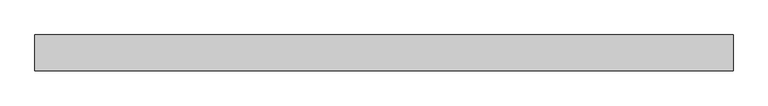
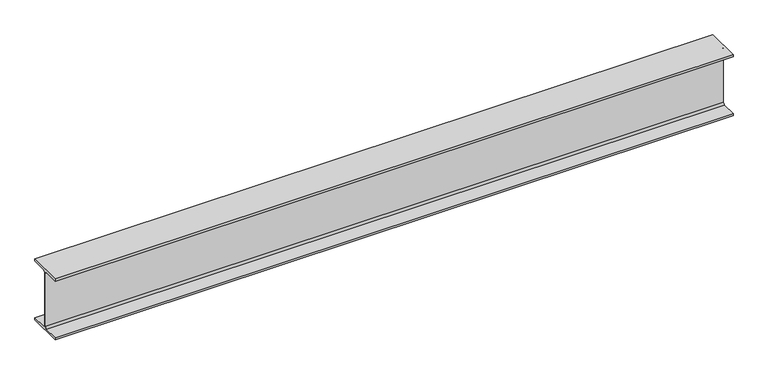
"""IFC4 building model written with IfcOpenShell, lengths in millimetres: beam geometry, Steel Beam_H-KSD3502 : H_SB_ASB_H-200x200x8x12."""

import ifcopenshell
import ifcopenshell.guid

model = None  # the IFC model being written
_history = None  # IfcOwnerHistory: only IFC2X3 demands one
_inside = {}  # id of a spatial element -> (the spatial element, [elements in it])
_under = {}  # id of a project, library or spatial element -> (it, [spatial elements below it])
_declared = {}  # id of a project -> (the project, [libraries it declares])
_typed = {}  # id of a type object -> (the type object, [elements of that type])
_made_of = {}  # id of a material, layer set ... -> (it, [elements and type objects made of it])


def new_model(schema):
    """Start an empty IFC model of exactly this schema.

    Asked for "IFC4X3", IfcOpenShell would pick the latest addendum, in which some entities
    have other attributes; the version numbers below select the first issue.
    IFC2X3 requires an IfcOwnerHistory on every rooted entity: one is made here for all.
    """
    global model, _history
    if schema == "IFC4X3":
        model = ifcopenshell.file(schema_version=(4, 3, 0, 0))
    else:
        model = ifcopenshell.file(schema=schema)
    _inside.clear()
    _under.clear()
    _declared.clear()
    _typed.clear()
    _made_of.clear()
    _history = None
    if model.schema == "IFC2X3":
        org = make("IfcOrganization", Name="unknown")
        user = make(
            "IfcPersonAndOrganization",
            ThePerson=make("IfcPerson", FamilyName="unknown"),
            TheOrganization=org,
        )
        app = make(
            "IfcApplication",
            ApplicationDeveloper=org,
            Version="unknown",
            ApplicationFullName="unknown",
            ApplicationIdentifier="unknown",
        )
        _history = make(
            "IfcOwnerHistory",
            OwningUser=user,
            OwningApplication=app,
            ChangeAction="ADDED",
            CreationDate=0,
        )
    return model


def make(cls, **values):
    """One entity of the class cls with the attributes given. An attribute that is None is left unset."""
    return model.create_entity(
        cls, **{name: value for name, value in values.items() if value is not None}
    )


def rooted(cls, **values):
    """An entity with a GlobalId (a new one), such as an element, a storey or a relation."""
    return make(cls, GlobalId=ifcopenshell.guid.new(), OwnerHistory=_history, **values)


def si_unit(unit_type, name, prefix=None):
    """IfcSIUnit, for example si_unit("LENGTHUNIT", "METRE", prefix="MILLI")."""
    return make("IfcSIUnit", UnitType=unit_type, Prefix=prefix, Name=name)


def assignment(units):
    """IfcUnitAssignment: the units of a project."""
    return None if units is None else make("IfcUnitAssignment", Units=units)


def point(xyz):
    """IfcCartesianPoint."""
    return None if xyz is None else make("IfcCartesianPoint", Coordinates=xyz)


def direction(xyz):
    """IfcDirection."""
    return None if xyz is None else make("IfcDirection", DirectionRatios=xyz)


def frame(location, z_axis=None, x_axis=None):
    """IfcAxis2Placement3D, a coordinate frame: its origin and axes. An axis left out is left unset."""
    return make(
        "IfcAxis2Placement3D",
        Location=point(location),
        Axis=direction(z_axis),
        RefDirection=direction(x_axis),
    )


def frame_2d(location, x_axis=None):
    """IfcAxis2Placement2D, a coordinate frame in the plane: its origin and x axis."""
    return make(
        "IfcAxis2Placement2D", Location=point(location), RefDirection=direction(x_axis)
    )


def origin():
    """The frame at (0, 0, 0) with its axes left unset."""
    return frame((0.0, 0.0, 0.0))


def place(relative_to, where):
    """IfcLocalPlacement: puts the frame where relative to a parent placement (None: the world)."""
    return make(
        "IfcLocalPlacement", PlacementRelTo=relative_to, RelativePlacement=where
    )


def context(
    kind, dimensions, precision=None, world=None, true_north=None, identifier=None
):
    """IfcGeometricRepresentationContext, for example the 3D "Model" context."""
    return make(
        "IfcGeometricRepresentationContext",
        ContextIdentifier=identifier,
        ContextType=kind,
        CoordinateSpaceDimension=dimensions,
        Precision=precision,
        WorldCoordinateSystem=world,
        TrueNorth=true_north,
    )


def project(units=None, contexts=None):
    """IfcProject with its units and contexts."""
    return rooted(
        "IfcProject",
        Name="project",
        RepresentationContexts=contexts,
        UnitsInContext=assignment(units),
    )


def spatial(cls, under=None, at=None, **own):
    """A site, building, storey or space (cls), placed at a placement, below another one or the project."""
    s = rooted(cls, ObjectPlacement=at, **own)
    if under is not None:
        _under.setdefault(under.id(), (under, []))[1].append(s)
    return s


def polyline(points):
    """IfcPolyline through the points."""
    return make("IfcPolyline", Points=[point(p) for p in points])


def circle_curve(where, radius):
    """IfcCircle in the frame where."""
    return make("IfcCircle", Position=where, Radius=radius)


def trimmed(basis, trim1, trim2, sense, master):
    """IfcTrimmedCurve: the piece of a basis curve between two trims."""
    return make(
        "IfcTrimmedCurve",
        BasisCurve=basis,
        Trim1=trim1,
        Trim2=trim2,
        SenseAgreement=sense,
        MasterRepresentation=master,
    )


def segment(curve, same_sense, transition):
    """IfcCompositeCurveSegment."""
    return make(
        "IfcCompositeCurveSegment",
        Transition=transition,
        SameSense=same_sense,
        ParentCurve=curve,
    )


def composite_curve(segments, self_intersect=None):
    """IfcCompositeCurve: segments joined end to end."""
    return make("IfcCompositeCurve", Segments=segments, SelfIntersect=self_intersect)


def outline(outer, holes=None, kind="AREA"):
    """IfcArbitraryClosedProfileDef: a profile drawn as a closed curve; with holes, ...WithVoids."""
    if holes is None:
        return make("IfcArbitraryClosedProfileDef", ProfileType=kind, OuterCurve=outer)
    return make(
        "IfcArbitraryProfileDefWithVoids",
        ProfileType=kind,
        OuterCurve=outer,
        InnerCurves=holes,
    )


def extrude(swept, where, along, depth):
    """IfcExtrudedAreaSolid: the profile swept, set in the frame where, extruded along a direction by depth."""
    return make(
        "IfcExtrudedAreaSolid",
        SweptArea=swept,
        Position=where,
        ExtrudedDirection=direction(along),
        Depth=depth,
    )


def shape(context_of_items, identifier, shape_type, items):
    """IfcShapeRepresentation: the items that make up one representation, for example the "Body"."""
    return make(
        "IfcShapeRepresentation",
        ContextOfItems=context_of_items,
        RepresentationIdentifier=identifier,
        RepresentationType=shape_type,
        Items=items,
    )


def source(mapping_origin, context_of_items, identifier, shape_type, items):
    """IfcRepresentationMap: a shape defined once, which mapped items show again and again."""
    return make(
        "IfcRepresentationMap",
        MappingOrigin=mapping_origin,
        MappedRepresentation=shape(context_of_items, identifier, shape_type, items),
    )


def transform(
    local_origin,
    x_axis=None,
    y_axis=None,
    z_axis=None,
    scale=None,
    scale2=None,
    scale3=None,
    uniform=True,
):
    """IfcCartesianTransformationOperator3D, or its non-uniform kind. x_axis, y_axis, z_axis: its Axis1, 2, 3."""
    if uniform:
        return make(
            "IfcCartesianTransformationOperator3D",
            Axis1=direction(x_axis),
            Axis2=direction(y_axis),
            LocalOrigin=point(local_origin),
            Scale=scale,
            Axis3=direction(z_axis),
        )
    return make(
        "IfcCartesianTransformationOperator3DnonUniform",
        Axis1=direction(x_axis),
        Axis2=direction(y_axis),
        LocalOrigin=point(local_origin),
        Scale=scale,
        Axis3=direction(z_axis),
        Scale2=scale2,
        Scale3=scale3,
    )


def mapped(mapping_source, mapping_target):
    """IfcMappedItem: shows the shape of a source again, moved by a transform."""
    return make(
        "IfcMappedItem", MappingSource=mapping_source, MappingTarget=mapping_target
    )


def made_of(thing, what):
    """Note that an element or type object is made of a material, layer set ...; save() writes the relation."""
    if what is not None:
        _made_of.setdefault(what.id(), (what, []))[1].append(thing)
    return thing


def element(
    cls,
    number,
    at=None,
    inside=None,
    cuts=None,
    type_object=None,
    material=None,
    context=None,
    identifier="Body",
    shape_type=None,
    held_by="IfcProductDefinitionShape",
    body=None,
    shapes=None,
    **own,
):
    """One element of the class cls, such as IfcWall. Its Tag is "e" and its number.

    at: its placement. inside: the storey or other place that contains it. cuts: it is an
    opening in that element (IfcRelVoidsElement). A single representation is given by context,
    identifier, shape_type and body (its items); several are given by shapes. held_by: the class
    of the entity that holds the representations. save() writes the other relations.
    """
    e = rooted(cls, Tag="e%d" % number, ObjectPlacement=at, **own)
    if body is not None:
        shapes = [shape(context, identifier, shape_type, body)]
    if shapes is not None:
        e.Representation = make(held_by, Representations=shapes)
    if inside is not None:
        _inside.setdefault(inside.id(), (inside, []))[1].append(e)
    if cuts is not None:
        rooted(
            "IfcRelVoidsElement", RelatingBuildingElement=cuts, RelatedOpeningElement=e
        )
    if type_object is not None:
        _typed.setdefault(type_object.id(), (type_object, []))[1].append(e)
    return made_of(e, material)


def aggregate(whole, parts):
    """IfcRelAggregates: a whole, such as a stair, and the parts it consists of."""
    return rooted("IfcRelAggregates", RelatingObject=whole, RelatedObjects=parts)


def save(model, path):
    """Write the relations noted so far, then the file.

    IfcRelAggregates (storeys below a building ...), IfcRelContainedInSpatialStructure (elements
    in a storey), IfcRelDefinesByType, IfcRelAssociatesMaterial and IfcRelDeclares: one each for
    every whole, place, type object, material and project.
    """
    for whole, parts in _under.values():
        aggregate(whole, parts)
    for where, things in _inside.values():
        rooted(
            "IfcRelContainedInSpatialStructure",
            RelatedElements=things,
            RelatingStructure=where,
        )
    for kind, things in _typed.values():
        rooted("IfcRelDefinesByType", RelatedObjects=things, RelatingType=kind)
    for what, things in _made_of.values():
        rooted("IfcRelAssociatesMaterial", RelatedObjects=things, RelatingMaterial=what)
    for by, libraries in _declared.values():
        rooted("IfcRelDeclares", RelatingContext=by, RelatedDefinitions=libraries)
    model.write(path)


def beam_0bb79bd1(model_context):
    return source(origin(), model_context, "Body", "SweptSolid", [
        extrude(outline(composite_curve([segment(polyline([(82.5, -141.5), (82.5, -151.7), (-82.5, -151.7), (-82.5, -141.5), (-11.9, -141.5)]), True, "CONTINUOUS"), segment(trimmed(circle_curve(frame_2d((-11.9, -132.6)), 8.9), [point((-11.9, -141.5))], [point((-3.0, -132.6))], True, "CARTESIAN"), True, "CONTINUOUS"), segment(polyline([(-3.0, -132.6), (-3.0, 132.6)]), True, "CONTINUOUS"), segment(trimmed(circle_curve(frame_2d((-11.9, 132.6)), 8.9), [point((-3.0, 132.6))], [point((-11.9, 141.5))], True, "CARTESIAN"), True, "CONTINUOUS"), segment(polyline([(-11.9, 141.5), (-82.5, 141.5), (-82.5, 151.7), (82.5, 151.7), (82.5, 141.5), (11.9, 141.5)]), True, "CONTINUOUS"), segment(trimmed(circle_curve(frame_2d((11.9, 132.6)), 8.9), [point((11.9, 141.5))], [point((3.0, 132.6))], True, "CARTESIAN"), True, "CONTINUOUS"), segment(polyline([(3.0, 132.6), (3.0, -132.6)]), True, "CONTINUOUS"), segment(trimmed(circle_curve(frame_2d((11.9, -132.6)), 8.9), [point((3.0, -132.6))], [point((11.9, -141.5))], True, "CARTESIAN"), True, "CONTINUOUS"), segment(polyline([(11.9, -141.5), (82.5, -141.5)]), True, "CONTINUOUS")], self_intersect=False)), frame((-1390.503051, 0.0, 0.0), z_axis=(1.0, 0.0, 0.0), x_axis=(0.0, 1.0, 0.0)), (0.0, 0.0, 1.0), 3204.7445716),
    ])


if __name__ == "__main__":
    model = new_model("IFC4")
    model_context = context("Model", 3, world=origin())
    ifc_project = project(units=[si_unit("LENGTHUNIT", "METRE", prefix="MILLI")], contexts=[model_context])
    site = spatial("IfcSite", under=ifc_project)
    building = spatial("IfcBuilding", under=site)
    placement = place(None, origin())
    beam_shape = beam_0bb79bd1(model_context)
    element("IfcBeam", 1, ObjectType="Steel Beam_H-KSD3502 : H_SB_ASB_H-200x200x8x12", at=placement, inside=building, context=model_context, shape_type="MappedRepresentation", body=[
        mapped(beam_shape, transform((0.0, 0.0, 0.0), x_axis=(1.0, 0.0, 0.0), y_axis=(0.0, 1.0, 0.0), z_axis=(0.0, 0.0, 1.0))),
    ])
    save(model, "model.ifc")

# Revit data of these elements
# Type "Steel Beam_H-KSD3502 : H_SB_ASB_H-200x200x8x12"
#   Width = 20.0 cm
#   Web Thickness = 0.8 cm
#   Web Fillet = 1.3 cm
#   Warping Constant = 141376.0 cm⁶
#   Torsional Moment of Inertia = 26.2485 cm⁴
#   Torsional Modulus = 1.0 cm³
#   Section Area = 63.53 cm²
#   Plastic Modulus weak axis = 244.0 cm³
#   Plastic Modulus strong axis = 525.0 cm³
#   Perimeter = 1.16 m²/m
#   Nominal Weight = 49.90 kgf/m
#   Moment of Inertia weak axis = 1600.00 cm⁴
#   Moment of Inertia strong axis = 4720.00 cm⁴
#   Height = 20.0 cm
#   Flange Thickness = 1.2 cm
#   Elastic Modulus weak axis = 160.0 cm³
#   Elastic Modulus strong axis = 472.0 cm³
#   Centroid Vertical = 10.0 cm
#   Centroid Horizontal = 10.0 cm
#   Length [instance default] = 1.5240 m
#   Structural Material [instance default] = Steel, 45-345
#   Assembly Code = ""
# Element 1 (IfcBeam, "Steel Beam_H-KSD3502 : H_SB_ASB_H-200x200x8x12")
#   Structural Material = none
# Materials
#   "Steel, 45-345": class "Metal", colour RGB 189 187 185, transparency 0, Description = "Steel 345 MPa", Cost = 0
